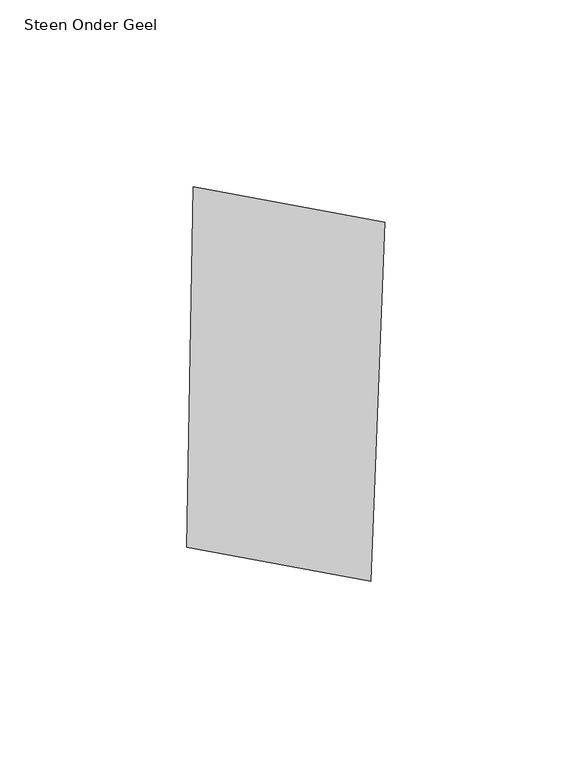
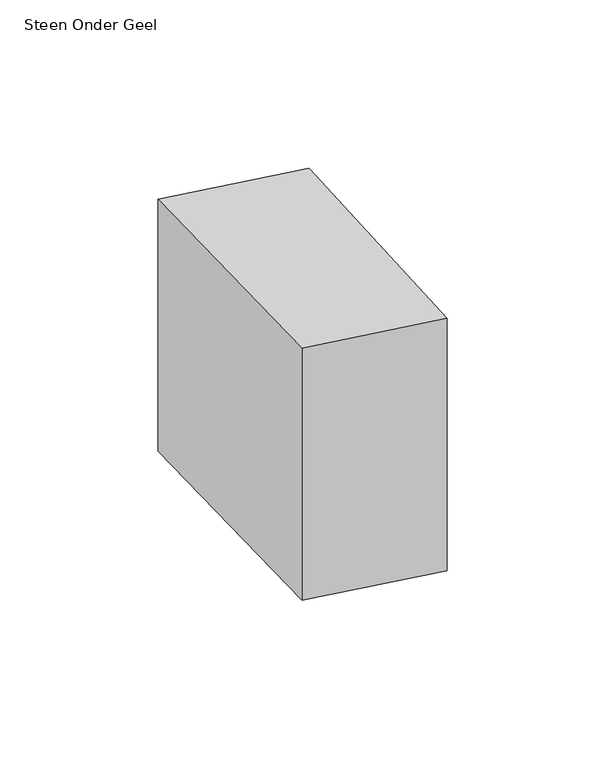
"""IFC4 building model written with IfcOpenShell, lengths in millimetres: proxy geometry, 00_GMA_steen_versie_4 : Steen Onder Geel."""

import ifcopenshell
import ifcopenshell.guid

model = None  # the IFC model being written
_history = None  # IfcOwnerHistory: only IFC2X3 demands one
_inside = {}  # id of a spatial element -> (the spatial element, [elements in it])
_under = {}  # id of a project, library or spatial element -> (it, [spatial elements below it])
_declared = {}  # id of a project -> (the project, [libraries it declares])
_typed = {}  # id of a type object -> (the type object, [elements of that type])
_made_of = {}  # id of a material, layer set ... -> (it, [elements and type objects made of it])


def new_model(schema):
    """Start an empty IFC model of exactly this schema.

    Asked for "IFC4X3", IfcOpenShell would pick the latest addendum, in which some entities
    have other attributes; the version numbers below select the first issue.
    IFC2X3 requires an IfcOwnerHistory on every rooted entity: one is made here for all.
    """
    global model, _history
    if schema == "IFC4X3":
        model = ifcopenshell.file(schema_version=(4, 3, 0, 0))
    else:
        model = ifcopenshell.file(schema=schema)
    _inside.clear()
    _under.clear()
    _declared.clear()
    _typed.clear()
    _made_of.clear()
    _history = None
    if model.schema == "IFC2X3":
        org = make("IfcOrganization", Name="unknown")
        user = make(
            "IfcPersonAndOrganization",
            ThePerson=make("IfcPerson", FamilyName="unknown"),
            TheOrganization=org,
        )
        app = make(
            "IfcApplication",
            ApplicationDeveloper=org,
            Version="unknown",
            ApplicationFullName="unknown",
            ApplicationIdentifier="unknown",
        )
        _history = make(
            "IfcOwnerHistory",
            OwningUser=user,
            OwningApplication=app,
            ChangeAction="ADDED",
            CreationDate=0,
        )
    return model


def make(cls, **values):
    """One entity of the class cls with the attributes given. An attribute that is None is left unset."""
    return model.create_entity(
        cls, **{name: value for name, value in values.items() if value is not None}
    )


def rooted(cls, **values):
    """An entity with a GlobalId (a new one), such as an element, a storey or a relation."""
    return make(cls, GlobalId=ifcopenshell.guid.new(), OwnerHistory=_history, **values)


def si_unit(unit_type, name, prefix=None):
    """IfcSIUnit, for example si_unit("LENGTHUNIT", "METRE", prefix="MILLI")."""
    return make("IfcSIUnit", UnitType=unit_type, Prefix=prefix, Name=name)


def assignment(units):
    """IfcUnitAssignment: the units of a project."""
    return None if units is None else make("IfcUnitAssignment", Units=units)


def point(xyz):
    """IfcCartesianPoint."""
    return None if xyz is None else make("IfcCartesianPoint", Coordinates=xyz)


def direction(xyz):
    """IfcDirection."""
    return None if xyz is None else make("IfcDirection", DirectionRatios=xyz)


def frame(location, z_axis=None, x_axis=None):
    """IfcAxis2Placement3D, a coordinate frame: its origin and axes. An axis left out is left unset."""
    return make(
        "IfcAxis2Placement3D",
        Location=point(location),
        Axis=direction(z_axis),
        RefDirection=direction(x_axis),
    )


def origin():
    """The frame at (0, 0, 0) with its axes left unset."""
    return frame((0.0, 0.0, 0.0))


def origin_with_axes():
    """The frame at (0, 0, 0) with the z axis (0, 0, 1) and the x axis (1, 0, 0) written out."""
    return frame((0.0, 0.0, 0.0), z_axis=(0.0, 0.0, 1.0), x_axis=(1.0, 0.0, 0.0))


def place(relative_to, where):
    """IfcLocalPlacement: puts the frame where relative to a parent placement (None: the world)."""
    return make(
        "IfcLocalPlacement", PlacementRelTo=relative_to, RelativePlacement=where
    )


def context(
    kind, dimensions, precision=None, world=None, true_north=None, identifier=None
):
    """IfcGeometricRepresentationContext, for example the 3D "Model" context."""
    return make(
        "IfcGeometricRepresentationContext",
        ContextIdentifier=identifier,
        ContextType=kind,
        CoordinateSpaceDimension=dimensions,
        Precision=precision,
        WorldCoordinateSystem=world,
        TrueNorth=true_north,
    )


def project(units=None, contexts=None):
    """IfcProject with its units and contexts."""
    return rooted(
        "IfcProject",
        Name="project",
        RepresentationContexts=contexts,
        UnitsInContext=assignment(units),
    )


def spatial(cls, under=None, at=None, **own):
    """A site, building, storey or space (cls), placed at a placement, below another one or the project."""
    s = rooted(cls, ObjectPlacement=at, **own)
    if under is not None:
        _under.setdefault(under.id(), (under, []))[1].append(s)
    return s


def polyline(points):
    """IfcPolyline through the points."""
    return make("IfcPolyline", Points=[point(p) for p in points])


def outline(outer, holes=None, kind="AREA"):
    """IfcArbitraryClosedProfileDef: a profile drawn as a closed curve; with holes, ...WithVoids."""
    if holes is None:
        return make("IfcArbitraryClosedProfileDef", ProfileType=kind, OuterCurve=outer)
    return make(
        "IfcArbitraryProfileDefWithVoids",
        ProfileType=kind,
        OuterCurve=outer,
        InnerCurves=holes,
    )


def extrude(swept, where, along, depth):
    """IfcExtrudedAreaSolid: the profile swept, set in the frame where, extruded along a direction by depth."""
    return make(
        "IfcExtrudedAreaSolid",
        SweptArea=swept,
        Position=where,
        ExtrudedDirection=direction(along),
        Depth=depth,
    )


def shape(context_of_items, identifier, shape_type, items):
    """IfcShapeRepresentation: the items that make up one representation, for example the "Body"."""
    return make(
        "IfcShapeRepresentation",
        ContextOfItems=context_of_items,
        RepresentationIdentifier=identifier,
        RepresentationType=shape_type,
        Items=items,
    )


def source(mapping_origin, context_of_items, identifier, shape_type, items):
    """IfcRepresentationMap: a shape defined once, which mapped items show again and again."""
    return make(
        "IfcRepresentationMap",
        MappingOrigin=mapping_origin,
        MappedRepresentation=shape(context_of_items, identifier, shape_type, items),
    )


def transform(
    local_origin,
    x_axis=None,
    y_axis=None,
    z_axis=None,
    scale=None,
    scale2=None,
    scale3=None,
    uniform=True,
):
    """IfcCartesianTransformationOperator3D, or its non-uniform kind. x_axis, y_axis, z_axis: its Axis1, 2, 3."""
    if uniform:
        return make(
            "IfcCartesianTransformationOperator3D",
            Axis1=direction(x_axis),
            Axis2=direction(y_axis),
            LocalOrigin=point(local_origin),
            Scale=scale,
            Axis3=direction(z_axis),
        )
    return make(
        "IfcCartesianTransformationOperator3DnonUniform",
        Axis1=direction(x_axis),
        Axis2=direction(y_axis),
        LocalOrigin=point(local_origin),
        Scale=scale,
        Axis3=direction(z_axis),
        Scale2=scale2,
        Scale3=scale3,
    )


def mapped(mapping_source, mapping_target):
    """IfcMappedItem: shows the shape of a source again, moved by a transform."""
    return make(
        "IfcMappedItem", MappingSource=mapping_source, MappingTarget=mapping_target
    )


def made_of(thing, what):
    """Note that an element or type object is made of a material, layer set ...; save() writes the relation."""
    if what is not None:
        _made_of.setdefault(what.id(), (what, []))[1].append(thing)
    return thing


def element(
    cls,
    number,
    at=None,
    inside=None,
    cuts=None,
    type_object=None,
    material=None,
    context=None,
    identifier="Body",
    shape_type=None,
    held_by="IfcProductDefinitionShape",
    body=None,
    shapes=None,
    **own,
):
    """One element of the class cls, such as IfcWall. Its Tag is "e" and its number.

    at: its placement. inside: the storey or other place that contains it. cuts: it is an
    opening in that element (IfcRelVoidsElement). A single representation is given by context,
    identifier, shape_type and body (its items); several are given by shapes. held_by: the class
    of the entity that holds the representations. save() writes the other relations.
    """
    e = rooted(cls, Tag="e%d" % number, ObjectPlacement=at, **own)
    if body is not None:
        shapes = [shape(context, identifier, shape_type, body)]
    if shapes is not None:
        e.Representation = make(held_by, Representations=shapes)
    if inside is not None:
        _inside.setdefault(inside.id(), (inside, []))[1].append(e)
    if cuts is not None:
        rooted(
            "IfcRelVoidsElement", RelatingBuildingElement=cuts, RelatedOpeningElement=e
        )
    if type_object is not None:
        _typed.setdefault(type_object.id(), (type_object, []))[1].append(e)
    return made_of(e, material)


def aggregate(whole, parts):
    """IfcRelAggregates: a whole, such as a stair, and the parts it consists of."""
    return rooted("IfcRelAggregates", RelatingObject=whole, RelatedObjects=parts)


def save(model, path):
    """Write the relations noted so far, then the file.

    IfcRelAggregates (storeys below a building ...), IfcRelContainedInSpatialStructure (elements
    in a storey), IfcRelDefinesByType, IfcRelAssociatesMaterial and IfcRelDeclares: one each for
    every whole, place, type object, material and project.
    """
    for whole, parts in _under.values():
        aggregate(whole, parts)
    for where, things in _inside.values():
        rooted(
            "IfcRelContainedInSpatialStructure",
            RelatedElements=things,
            RelatingStructure=where,
        )
    for kind, things in _typed.values():
        rooted("IfcRelDefinesByType", RelatedObjects=things, RelatingType=kind)
    for what, things in _made_of.values():
        rooted("IfcRelAssociatesMaterial", RelatedObjects=things, RelatingMaterial=what)
    for by, libraries in _declared.values():
        rooted("IfcRelDeclares", RelatingContext=by, RelatedDefinitions=libraries)
    model.write(path)


def steen_onder_geel_38020695(model_context):
    return source(origin(), model_context, "Body", "SweptSolid", [
        extrude(outline(polyline([(102.3943772, 114.9879868), (98.6843103, 19.0205222), (49.5109476, 28.074825), (51.1434833, 124.4390492), (102.3943772, 114.9879868)])), origin_with_axes(), (0.0, 0.0, 1.0), 100.0),
    ])


if __name__ == "__main__":
    model = new_model("IFC4")
    model_context = context("Model", 3, world=origin())
    ifc_project = project(units=[si_unit("LENGTHUNIT", "METRE", prefix="MILLI")], contexts=[model_context])
    site = spatial("IfcSite", under=ifc_project)
    building = spatial("IfcBuilding", under=site)
    placement = place(None, origin())
    steen_onder_geel_shape = steen_onder_geel_38020695(model_context)
    element("IfcBuildingElementProxy", 1, Name="00_GMA_steen_versie_4 : Steen Onder Geel", ObjectType="00_GMA_steen_versie_4 : Steen Onder Geel", at=placement, inside=building, context=model_context, shape_type="MappedRepresentation", body=[
        mapped(steen_onder_geel_shape, transform((0.0, 0.0, 0.0), x_axis=(1.0, 0.0, 0.0), y_axis=(0.0, 1.0, 0.0), z_axis=(0.0, 0.0, 1.0))),
    ])
    save(model, "model.ifc")

# Revit data of these elements
# Type "00_GMA_steen_versie_4 : Steen Onder Geel"
#   StootVoegHalfBoven [instance default] = 5 mm
#   StootVoegHalf [instance default] = 5 mm
#   StootVoegBreedteOnder = 10 mm
#   StootVoegBreedteBoven = 10 mm
#   Steendikte = 100 mm
#   LintVoegOnderHalf = 0 mm
#   LintVoegOnder = 0 mm
#   LintVoegBovenHalf = 5 mm
#   LintVoegBoven = 10 mm
#   materiaal = 21_steen_geel
#   MateriaalVoeg = none
#   Default Elevation = 0
# Element 1 (IfcBuildingElementProxy, "00_GMA_steen_versie_4 : Steen Onder Geel")
#   Materials on its faces: "21_steen_geel"
# Materials
#   "21_steen_geel": class "Unassigned", colour RGB 202 202 0, transparency 0, Cost = 0
